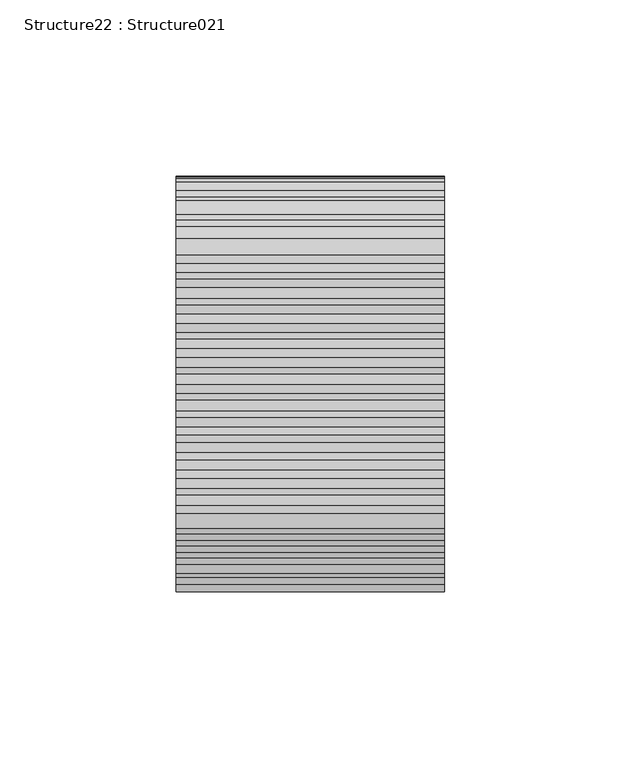
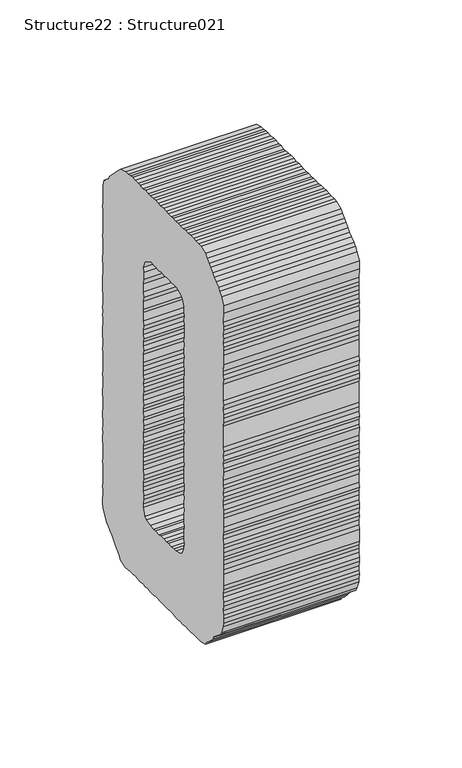
"""IFC4 building model written with IfcOpenShell, lengths in millimetres: proxy geometry, Structure22 : Structure021."""

from ifc_helpers import new_model, si_unit, frame, origin, place, context, project, spatial, polyline, outline, extrude, source, transform, mapped, element, save


def structure22_structure021_bf8fffc0(model_context):
    return source(origin(), model_context, "Body", "SweptSolid", [
        extrude(outline(polyline([(4.7286773, -1e-07), (6.3783559, -1.8768646), (9.1046649, -2.8984913), (12.8113915, -5.6317787), (15.1185363, -7.6753561), (16.8767637, -8.5970884), (19.0634231, -10.0418496), (21.7925729, -11.0775952), (23.432295, -12.9651048), (25.8559498, -17.1940296), (26.5970375, -19.2666708), (27.4444766, -21.9280094), (27.5109558, -23.8088696), (27.6872958, -26.2958687), (28.9086843, -29.2051618), (29.3991488, -31.6427836), (29.2748298, -34.1859564), (29.7626206, -36.6102896), (30.5010345, -38.6696421), (31.2876459, -41.0286658), (32.6920287, -48.0084865), (32.8818343, -50.502282), (33.42945, -53.223947), (34.2777246, -55.8894383), (34.3468776, -57.7835872), (35.1943167, -60.4449258), (35.6839456, -62.8783949), (35.8084116, -65.047451), (36.0472503, -67.8450703), (36.5368792, -70.2785395), (37.5732783, -72.2684298), (37.8237443, -75.0637096), (38.860989, -80.2188438), (39.7084281, -82.8801825), (39.8384086, -85.0766462), (40.0744065, -87.8601465), (40.5033749, -89.9921312), (41.6631003, -92.5949567), (41.4787892, -94.8399672), (42.3396939, -97.5081022), (42.3927076, -99.382166), (43.0038246, -102.4194345), (44.5915158, -107.1492616), (44.6588306, -109.0342745), (44.8948284, -111.8177748), (45.9332328, -113.8176315), (45.8115876, -116.3740928), (46.670654, -119.0330919), (46.8486651, -121.5283963), (49.2884543, -133.6542153), (50.3895245, -135.9655228), (50.9369731, -138.6863573), (51.0042879, -140.5713702), (51.2431265, -143.3689895), (52.4618414, -146.2649942), (52.2803712, -148.5241237), (54.2323697, -158.2256093), (55.091269, -160.883778), (55.2696143, -163.3807435), (55.7572379, -165.8042462), (57.2226055, -169.9261213), (58.3221817, -175.3910451), (58.5103161, -177.8765352), (59.2344289, -179.9249387), (59.0527916, -182.1832376), (59.9118581, -184.8422369), (60.0300442, -187.0402095), (60.8892777, -189.7000392), (61.316408, -191.8228881), (61.494419, -194.3181925), (63.2009246, -199.6385304), (64.1183522, -204.1981705), (62.788769, -208.567853), (61.3937043, -211.0573386), (60.4855896, -212.8102336), (58.4308862, -215.1222095), (56.9116645, -216.9989271), (55.707231, -218.8252697), (54.3113356, -221.3149225), (53.1052309, -223.1329598), (51.6518451, -225.3325886), (50.4932744, -227.4512948), (46.5548849, -229.8285903), (44.4926916, -230.5528851), (41.4587453, -231.1633338), (39.7081748, -231.8301131), (36.9748824, -232.3800684), (34.4913826, -232.5652099), (31.7572596, -233.1153323), (29.5754163, -233.2449636), (26.8529208, -233.7927465), (24.7782694, -234.5195479), (22.5964261, -234.6491793), (19.9337555, -235.4942939), (18.0517356, -235.563599), (15.0177892, -236.1740476), (13.2545887, -236.8381833), (10.8935747, -237.6277876), (7.7389758, -237.6385896), (6.0374333, -238.6048731), (3.3149378, -239.1526559), (0.8198105, -239.340137), (-1.9733069, -239.5927605), (-3.7847049, -239.9572249), (-6.0867245, -241.0443281), (-8.9406696, -240.9946366), (-11.2426892, -242.0817398), (-13.0648842, -242.4483767), (-16.1596581, -242.7565103), (-18.5215027, -243.5462818), (-20.3436976, -243.9129186), (-22.8870225, -243.8007285), (-25.3213221, -244.2905245), (-30.1724902, -243.6817419), (-34.117377, -241.3152484), (-36.3057075, -239.8621819), (-38.1927107, -238.3562638), (-42.8603983, -235.5026379), (-44.198626, -233.5631075), (-46.3242907, -232.4214918), (-49.1142681, -231.0834312), (-50.7588064, -227.6215291), (-51.6062454, -224.9601904), (-52.1538611, -222.2385254), (-52.3434996, -219.7455606), (-52.7704627, -217.6235422), (-53.8725355, -215.3072514), (-53.9878807, -213.1233978), (-54.4748359, -210.7032172), (-54.6628033, -208.2185577), (-55.2130928, -205.4836041), (-56.06237, -202.8131295), (-56.2501703, -200.3293006), (-57.2884075, -198.3302743), (-57.1669295, -195.7729826), (-58.6917978, -188.1943457), (-59.7273612, -186.208608), (-60.2776507, -183.4736545), (-60.333338, -181.5863021), (-60.9434525, -178.5540168), (-61.0707594, -176.3708417), (-62.1089966, -174.3718155), (-63.6338648, -166.7931786), (-63.6328723, -163.6370707), (-64.547459, -159.0915497), (-65.5877015, -157.0825571), (-65.884527, -153.9967419), (-66.563283, -152.2338905), (-66.7414611, -149.7377556), (-67.2282492, -147.3184055), (-68.0303316, -144.942619), (-69.0020696, -140.1130548), (-69.1800806, -137.6177504), (-69.6680385, -135.1925866), (-70.5896037, -132.2229671), (-70.7079568, -130.0241639), (-71.1947449, -127.6048139), (-71.3853861, -125.1068657), (-71.8705031, -122.6958211), (-72.7196132, -120.0261771), (-73.5215285, -117.651221), (-73.3345437, -115.4194992), (-74.2513029, -110.8631812), (-75.4100256, -108.2653388), (-75.8398295, -106.1292014), (-76.0759945, -103.3448706), (-77.1738996, -97.888252), (-77.9123135, -95.8288996), (-78.4001043, -93.4045663), (-78.5782824, -90.9084314), (-78.8287486, -88.1131515), (-79.864312, -86.1274139), (-79.8033274, -83.2694682), (-80.7809041, -81.5719264), (-81.270533, -79.1384573), (-81.2077102, -76.2896475), (-81.9346637, -74.2271249), (-82.9717412, -69.0728214), (-83.7074814, -67.0267574), (-83.8864951, -64.5264698), (-84.9835647, -59.0740039), (-85.1742059, -56.5760558), (-85.601169, -54.4540375), (-86.6993983, -52.156849), (-86.8149106, -49.9721649), (-87.0047162, -47.4783695), (-88.103781, -45.1770283), (-88.6513967, -42.4553634), (-88.8902354, -39.657744), (-87.8014812, -35.6458867), (-86.7766946, -32.9223985), (-85.2609772, -31.0325596), (-84.0540419, -29.2143551), (-82.5383246, -27.3245161), (-80.8397651, -24.7886561), (-79.6961591, -22.6599985), (-77.0207013, -18.657267), (-75.9370873, -16.2304472), (-71.9986978, -13.8531517), (-69.201909, -13.6144802), (-66.7194119, -13.4243553), (-64.6572186, -12.7000606), (-62.4745447, -12.570262), (-59.8118741, -11.7251476), (-57.6782283, -11.2958449), (-54.5844571, -10.9827279), (-52.8337145, -10.321099), (-50.0397665, -10.0683083), (-48.0394085, -9.0323956), (-45.6175669, -8.5451062), (-43.0607764, -8.6640926), (-40.938758, -8.2371295), (-38.2760875, -7.392015), (-30.9856465, -5.9251335), (-28.5147768, -5.7373482), (-26.0813077, -5.2477193), (-23.7811263, -4.1514802), (-21.659108, -3.7245171), (-19.4619658, -3.6064982), (-16.8021361, -2.7472645), (-13.9463529, -2.8060918), (-11.8833289, -2.08163), (-9.4606567, -1.5941734), (-6.6675394, -1.3415499), (-4.2448672, -0.8540933), (-2.1826738, -0.1297986), (0.0, 0.0), (4.7286773, -1e-07)]), holes=[polyline([(-13.4242219, -199.9211019), (-8.7405971, -201.1875179), (-6.3787475, -200.4020662), (-4.1959065, -200.2730982), (-1.8955581, -199.1776897), (0.6602348, -199.2960128), (2.9605833, -198.2006042), (5.5047486, -198.3212669), (7.9274208, -197.8338103), (10.6015517, -196.9855257), (12.7835621, -196.8567249), (15.2178618, -196.3669288), (19.0847989, -193.6946411), (20.0010367, -191.9262852), (20.8415022, -188.2867164), (20.2313878, -185.2544311), (20.3550383, -182.7079363), (19.6280848, -180.6454137), (19.3776186, -177.8501338), (17.9160846, -170.58627), (16.9358341, -168.8754397), (16.9388321, -165.7292981), (15.8396001, -163.4271264), (15.7849154, -161.5447572), (15.4736217, -158.4471624), (14.4335462, -156.4390004), (14.0084213, -154.3261179), (14.009581, -151.1708406), (13.57961, -149.0338726), (12.4208872, -146.4360303), (12.2453829, -143.9531839), (11.5667938, -142.1911631), (11.4511145, -140.0056484), (10.6502018, -137.6356757), (10.7140274, -134.7918491), (9.8664213, -132.1296799), (8.9498292, -127.5741924), (8.1505876, -125.212525), (8.2115723, -122.3545794), (6.6230456, -117.6205996), (6.7473646, -115.0774269), (5.771626, -113.389021), (5.5327874, -110.5914016), (5.4056476, -108.409057), (4.3047445, -106.09858), (4.1284046, -103.6115809), (3.5182902, -100.5792956), (2.8405367, -98.8214276), (2.9640202, -96.2741021), (1.8051303, -93.6754293), (1.749443, -91.7880769), (0.7105273, -86.6246374), (0.5225598, -84.1399778), (-0.0250559, -81.4183129), (-0.6920173, -79.6539525), (-0.9398097, -76.8719613), (-1.7265882, -74.5121071), (-2.4676759, -72.4394659), (-2.3441925, -69.8921406), (-3.1934697, -67.221666), (-4.1082235, -62.6753145), (-4.2980292, -60.181519), (-5.1454682, -57.5201803), (-5.6939194, -54.7943627), (-6.3743467, -53.023206), (-6.3106882, -50.1785489), (-7.1581272, -47.5172102), (-9.4166083, -44.1693314), (-11.1809536, -43.2730265), (-15.5973446, -43.2145134), (-17.7828592, -43.3301928), (-19.9048776, -43.7571559), (-22.5763347, -44.6187291), (-24.7610189, -44.7342413), (-27.1210253, -45.5331487), (-30.2176374, -45.8321465), (-32.100493, -45.8972989), (-35.0737787, -46.8092319), (-37.2572881, -46.9348778), (-39.8672542, -48.0977683), (-43.6291468, -49.8018022), (-44.5989245, -51.2482295), (-45.2537371, -55.8062035), (-44.826774, -57.9282219), (-43.979335, -60.5895605), (-43.549531, -62.725698), (-43.6615541, -65.2698533), (-42.814115, -67.9311919), (-42.3851466, -70.0631767), (-41.5976997, -72.4263531), (-41.1705694, -74.549202), (-41.1601017, -77.7021399), (-40.672311, -80.1264731), (-39.8846968, -82.4904801), (-39.6950584, -84.983445), (-39.2679282, -87.1062938), (-38.418818, -89.7759379), (-38.0543536, -91.5873359), (-37.2640658, -93.9646314), (-37.3767573, -96.5054646), (-36.5293182, -99.1668032), (-35.7998581, -101.2417839), (-35.3754016, -103.3513442), (-35.0642749, -106.4481084), (-34.3356503, -108.5189363), (-34.3876813, -111.3612538), (-34.0203761, -113.186771), (-32.9339413, -115.4854684), (-33.0457972, -118.0304543), (-32.4330091, -121.0760282), (-31.3455716, -123.3797088), (-30.8586165, -125.7998893), (-30.7913016, -127.6849022), (-29.9438626, -130.3462409), (-29.7542241, -132.8392059), (-29.2664333, -135.2635391), (-29.0793015, -137.744046), (-28.2273505, -140.4278092), (-27.3154375, -144.9600416), (-26.5858102, -147.0358527), (-26.6378412, -149.8781702), (-26.2080373, -152.0143077), (-25.1841012, -154.0023849), (-25.2961243, -156.5465402), (-24.8063282, -158.9808398), (-23.6592329, -161.5810217), (-23.7085902, -164.4366279), (-22.7311705, -169.2944302), (-22.0652116, -171.0538073), (-21.0902986, -175.8991517), (-20.3001779, -178.2756167), (-20.3522089, -181.1179342), (-19.3757919, -185.9707534), (-18.2275268, -188.576749), (-17.3736006, -192.8207857), (-17.4862921, -195.3616188), (-14.8216312, -199.2421887), (-13.4242219, -199.9211019)])]), frame((-35624.0862846, 276587.449163, 3983.4414729), z_axis=(1.0, 0.0, 1.3542500454377657e-12), x_axis=(0.0, -0.9803526236909532, 0.19725296758797886)), (0.0, 0.0, 1.0), 76.2),
    ])


if __name__ == "__main__":
    model = new_model("IFC4")
    model_context = context("Model", 3, world=origin())
    ifc_project = project(units=[si_unit("LENGTHUNIT", "METRE", prefix="MILLI")], contexts=[model_context])
    site = spatial("IfcSite", under=ifc_project)
    building = spatial("IfcBuilding", under=site)
    placement = place(None, origin())
    structure22_structure021_shape = structure22_structure021_bf8fffc0(model_context)
    element("IfcBuildingElementProxy", 1, Name="Structure22 : Structure021", ObjectType="Structure22 : Structure021", at=placement, inside=building, context=model_context, shape_type="MappedRepresentation", body=[
        mapped(structure22_structure021_shape, transform((0.0, 0.0, 0.0), x_axis=(1.0, 0.0, 0.0), y_axis=(0.0, 1.0, 0.0), z_axis=(0.0, 0.0, 1.0))),
    ])
    save(model, "model.ifc")

# Revit data of these elements
# Type "Structure22 : Structure021"
#   NameOverride = "Structure021"
# Element 1 (IfcBuildingElementProxy, "Structure22 : Structure021")
#   Materials on its faces: "BRUSHED ALUMINUM LETTERING"
# Materials
#   "BRUSHED ALUMINUM LETTERING": class "Unassigned", colour RGB 169 181 186, transparency 0, Cost = 0
